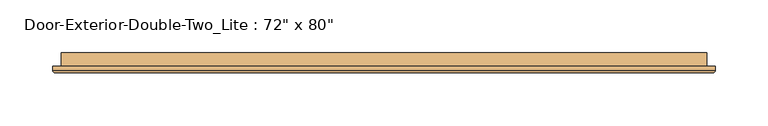
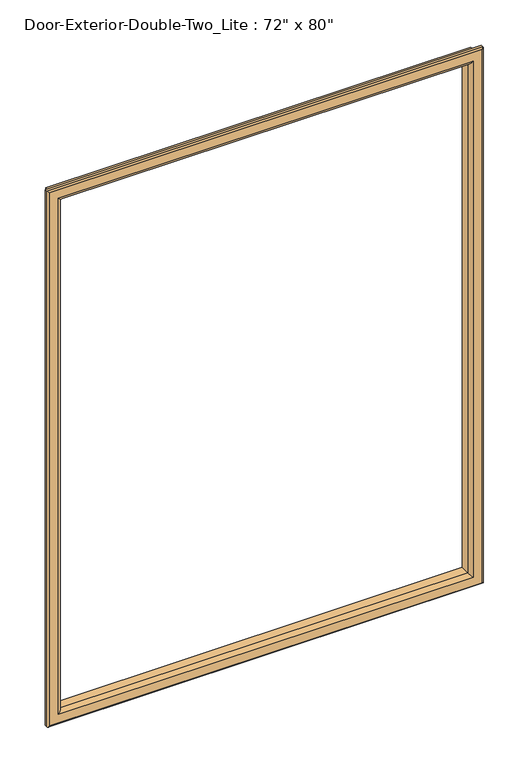
"""IFC4 building model written with IfcOpenShell, lengths in millimetres: door geometry."""

from ifc_helpers import new_model, si_unit, frame, origin, place, context, project, spatial, ellipse_curve, source, transform, mapped, element, save
from ifc_brep_helpers import plane_surface, cylinder_surface, advanced_brep


def door_3b4764fa(model_context):
    return source(origin(), model_context, "Body", "AdvancedBrep", [
        advanced_brep(
        [(-762.0, 47.625, 1117.6), (-762.0, 34.925, 1117.6), (-762.0, 34.925, 1914.525), (-762.0, 47.625, 1914.525), (-750.0, 33.925, 1129.6), (-750.0, 47.625, 1129.6), (-750.0, 47.625, 1902.525), (-750.0, 33.925, 1902.525), (-755.0, 28.925, 1124.6), (-755.0, 28.925, 1907.525), (-770.0, 30.925, 1109.6), (-768.0, 28.925, 1111.6), (-768.0, 28.925, 1920.525), (-770.0, 30.925, 1922.525), (-770.0, 34.925, 1109.6), (-770.0, 34.925, 1922.525), (-152.4, 34.925, 1914.525), (-152.4, 47.625, 1914.525), (-164.4, 47.625, 1902.525), (-164.4, 33.925, 1902.525), (-159.4, 28.925, 1907.525), (-146.4, 28.925, 1920.525), (-144.4, 30.925, 1922.525), (-144.4, 34.925, 1922.525), (-152.4, 34.925, 1117.6), (-152.4, 47.625, 1117.6), (-164.4, 47.625, 1129.6), (-164.4, 33.925, 1129.6), (-159.4, 28.925, 1124.6), (-146.4, 28.925, 1111.6), (-144.4, 30.925, 1109.6), (-144.4, 34.925, 1109.6)],
        [
            (0, 1),
            (1, 2),
            (2, 3),
            (3, 0),
            (4, 5),
            (5, 6),
            (6, 7),
            (7, 4),
            (8, 4, ellipse_curve(frame((-755.0, 33.925, 1124.6), z_axis=(-0.7071067811865475, 0.0, 0.7071067811865475), x_axis=(-0.7071067811865474, 0.0, -0.7071067811865476)), 7.0710678, 5.0)),
            (7, 9, ellipse_curve(frame((-755.0, 33.925, 1907.525), z_axis=(-0.7071067811865475, 0.0, -0.7071067811865475), x_axis=(0.7071067811865474, 0.0, -0.7071067811865476)), 7.0710678, 5.0)),
            (9, 8),
            (10, 11, ellipse_curve(frame((-768.0, 30.925, 1111.6), z_axis=(-0.7071067811865475, 0.0, 0.7071067811865475), x_axis=(-0.7071067811865474, 0.0, -0.7071067811865476)), 2.8284271, 2.0)),
            (11, 12),
            (12, 13, ellipse_curve(frame((-768.0, 30.925, 1920.525), z_axis=(-0.7071067811865475, 0.0, -0.7071067811865475), x_axis=(0.7071067811865474, 0.0, -0.7071067811865476)), 2.8284271, 2.0)),
            (13, 10),
            (14, 10),
            (13, 15),
            (15, 14),
            (2, 16),
            (16, 17),
            (17, 3),
            (6, 18),
            (18, 19),
            (19, 7),
            (19, 20, ellipse_curve(frame((-159.4, 33.925, 1907.525), z_axis=(-0.7071067811865475, 0.0, 0.7071067811865475), x_axis=(-0.7071067811865476, 0.0, -0.7071067811865474)), 7.0710678, 5.0)),
            (20, 9),
            (12, 21),
            (21, 22, ellipse_curve(frame((-146.4, 30.925, 1920.525), z_axis=(-0.7071067811865475, 0.0, 0.7071067811865475), x_axis=(-0.7071067811865476, 0.0, -0.7071067811865474)), 2.8284271, 2.0)),
            (22, 13),
            (22, 23),
            (23, 15),
            (16, 24),
            (24, 25),
            (25, 17),
            (18, 26),
            (26, 27),
            (27, 19),
            (27, 28, ellipse_curve(frame((-159.4, 33.925, 1124.6), z_axis=(0.7071067811865475, 0.0, 0.7071067811865475), x_axis=(-0.7071067811865474, 0.0, 0.7071067811865476)), 7.0710678, 5.0)),
            (28, 20),
            (21, 29),
            (29, 30, ellipse_curve(frame((-146.4, 30.925, 1111.6), z_axis=(0.7071067811865475, 0.0, 0.7071067811865475), x_axis=(-0.7071067811865474, 0.0, 0.7071067811865476)), 2.8284271, 2.0)),
            (30, 22),
            (30, 31),
            (31, 23),
            (31, 14),
            (1, 24),
            (0, 25),
            (5, 26),
            (4, 27),
            (8, 28),
            (11, 29),
            (10, 30),
        ],
        [
            plane_surface(frame((-762.0, 34.925, 1117.6), z_axis=(-1.0, 0.0, 0.0), x_axis=(0.0, 0.0, 1.0))),
            plane_surface(frame((-750.0, 47.625, 1129.6), z_axis=(1.0, 0.0, 0.0), x_axis=(0.0, 0.0, 1.0))),
            cylinder_surface(frame((-755.0, 33.925, 1117.6), z_axis=(0.0, 0.0, -1.0), x_axis=(-1.0, 0.0, 0.0)), 5.0),
            cylinder_surface(frame((-768.0, 30.925, 1117.6), z_axis=(0.0, 0.0, -1.0), x_axis=(-1.0, 0.0, 0.0)), 2.0),
            plane_surface(frame((-770.0, 30.925, 1109.6), z_axis=(-1.0, 0.0, 0.0), x_axis=(0.0, 0.0, 1.0))),
            plane_surface(frame((-762.0, 34.925, 1914.525), z_axis=(0.0, 0.0, 1.0), x_axis=(1.0, 0.0, 0.0))),
            plane_surface(frame((-750.0, 47.625, 1902.525), z_axis=(0.0, 0.0, -1.0), x_axis=(1.0, 0.0, 0.0))),
            cylinder_surface(frame((-762.0, 33.925, 1907.525), z_axis=(-1.0, 0.0, 0.0), x_axis=(0.0, 0.0, 1.0)), 5.0),
            cylinder_surface(frame((-762.0, 30.925, 1920.525), z_axis=(-1.0, 0.0, 0.0), x_axis=(0.0, 0.0, 1.0)), 2.0),
            plane_surface(frame((-770.0, 30.925, 1922.525), z_axis=(0.0, 0.0, 1.0), x_axis=(1.0, 0.0, 0.0))),
            plane_surface(frame((-152.4, 34.925, 1914.525), z_axis=(1.0, 0.0, 0.0), x_axis=(0.0, 0.0, -1.0))),
            plane_surface(frame((-164.4, 47.625, 1902.525), z_axis=(-1.0, 0.0, 0.0), x_axis=(0.0, 0.0, -1.0))),
            cylinder_surface(frame((-159.4, 33.925, 1914.525), z_axis=(0.0, 0.0, 1.0), x_axis=(1.0, 0.0, 0.0)), 5.0),
            cylinder_surface(frame((-146.4, 30.925, 1914.525), z_axis=(0.0, 0.0, 1.0), x_axis=(1.0, 0.0, 0.0)), 2.0),
            plane_surface(frame((-144.4, 30.925, 1922.525), z_axis=(1.0, 0.0, 0.0), x_axis=(0.0, 0.0, -1.0))),
            plane_surface(frame((-144.4, 34.925, 1109.6), z_axis=(0.0, 1.0, 0.0), x_axis=(-1.0, 0.0, 0.0))),
            plane_surface(frame((-152.4, 34.925, 1117.6), z_axis=(0.0, 0.0, -1.0), x_axis=(-1.0, 0.0, 0.0))),
            plane_surface(frame((-152.4, 47.625, 1117.6), z_axis=(0.0, 1.0, 0.0), x_axis=(-1.0, 0.0, 0.0))),
            plane_surface(frame((-164.4, 47.625, 1129.6), z_axis=(0.0, 0.0, 1.0), x_axis=(-1.0, 0.0, 0.0))),
            cylinder_surface(frame((-152.4, 33.925, 1124.6), z_axis=(1.0, 0.0, 0.0), x_axis=(0.0, 0.0, -1.0)), 5.0),
            plane_surface(frame((-159.4, 28.925, 1124.6), z_axis=(0.0, -1.0, 0.0), x_axis=(-1.0, 0.0, 0.0))),
            cylinder_surface(frame((-152.4, 30.925, 1111.6), z_axis=(1.0, 0.0, 0.0), x_axis=(0.0, 0.0, -1.0)), 2.0),
            plane_surface(frame((-144.4, 30.925, 1109.6), z_axis=(0.0, 0.0, -1.0), x_axis=(-1.0, 0.0, 0.0))),
        ],
        [
            (0, [[1, 2, 3, 4]]),
            (1, [[5, 6, 7, 8]]),
            (2, [[9, -8, 10, 11]]),
            (3, [[12, 13, 14, 15]]),
            (4, [[16, -15, 17, 18]]),
            (5, [[-3, 19, 20, 21]]),
            (6, [[-7, 22, 23, 24]]),
            (7, [[-10, -24, 25, 26]]),
            (8, [[-14, 27, 28, 29]]),
            (9, [[-17, -29, 30, 31]]),
            (10, [[-20, 32, 33, 34]]),
            (11, [[-23, 35, 36, 37]]),
            (12, [[-25, -37, 38, 39]]),
            (13, [[-28, 40, 41, 42]]),
            (14, [[-30, -42, 43, 44]]),
            (15, [[-31, -44, 45, -18], [46, -32, -19, -2]]),
            (16, [[-33, -46, -1, 47]]),
            (17, [[-21, -34, -47, -4], [48, -35, -22, -6]]),
            (18, [[-36, -48, -5, 49]]),
            (19, [[-38, -49, -9, 50]]),
            (20, [[51, -40, -27, -13], [-26, -39, -50, -11]]),
            (21, [[-41, -51, -12, 52]]),
            (22, [[-43, -52, -16, -45]]),
        ],
    ),
    ])


if __name__ == "__main__":
    model = new_model("IFC4")
    model_context = context("Model", 3, world=origin())
    ifc_project = project(units=[si_unit("LENGTHUNIT", "METRE", prefix="MILLI")], contexts=[model_context])
    site = spatial("IfcSite", under=ifc_project)
    building = spatial("IfcBuilding", under=site)
    placement = place(None, origin())
    door_shape = door_3b4764fa(model_context)
    element("IfcDoor", 1, ObjectType="Door-Exterior-Double-Two_Lite : 72\" x 80\"", at=placement, inside=building, context=model_context, shape_type="MappedRepresentation", body=[
        mapped(door_shape, transform((0.0, 0.0, 0.0), x_axis=(1.0, 0.0, 0.0), y_axis=(0.0, 1.0, 0.0), z_axis=(0.0, 0.0, 1.0))),
    ])
    save(model, "model.ifc")

# Revit data of these elements
# Type "Door-Exterior-Double-Two_Lite : 72\" x 80\""
#   Type Mark = "18"
#   Assembly Code = "B2030100"
#   Analytic Construction = "Metal frame, double glass door"
#   Top Rail = 0' - 4 5/8"
#   Threshold Length [instance default] = 6' - 4"
#   Threshold Offset [instance default] = 0' - 0 1/2"
#   Thickness = 0' - 1 3/4"
#   Thermal Resistance (R) = 0.242926 (m²·K)/W
#   Swing Angle [instance default] = 90.00°
#   Strike Height = 3' - 4"
#   Stiles = 0' - 6"
#   SinglePanelWidth = 3' - 0"
#   Rough Width [instance default] = 6' - 4"
#   Rough Height [instance default] = 7' - 0"
#   MFOpeningHeight [instance default] = 0' - 4"
#   MFOpeningWidth [instance default] = 0' - 4"
#   Lock Rail = 0' - 8"
#   Inset Calculate [instance default] = 0' - 4"
#   Masonry Inset [instance default] = 0' - 1"
#   Height = 6' - 8"
#   Width = 6' - 0"
#   Heat Transfer Coefficient (U) = 4.11674 W/(m²·K)
#   Glass Thickness = 0' - 0 3/4"
#   Masonry Frame Depth = 0' - 5 3/4"
#   Bottom Rail = 0' - 10"
#   Threshold [instance default] = yes
#   Masonry Frame [instance default] = yes
#   Function = 1
#   Dry Wall Frame [instance default] = no
#   Threshold Material = none
#   Panic Bar Material = Metal - Stainless Steel
#   Panel Material = Metal - Painted - Grey
#   Glass Stop Material = Metal - Painted - Grey
#   Frame Material = Metal - Painted - Grey
#   Exterior Pull Material = Metal - Stainless Steel
#   Visual Light Transmittance = 0
#   Solar Heat Gain Coefficient = 0
#   Wall Closure = (empty or 0)
# Element 1 (IfcDoor, "Door-Exterior-Double-Two_Lite : 72\" x 80\"")
#   Inset Calculate = 0' - 2 1/2"
#   Masonry Inset = -0' - 0 1/2"
#   Materials on its faces: "Metal - Painted - Grey", "Metal - Stainless Steel", "Glass"
# Materials
#   "Metal - Stainless Steel": class "Metal", colour RGB 247 247 247, transparency 0
#   "Metal - Painted - Grey": class "Paint", colour RGB 104 104 104, transparency 0, Cost = 0
#   "Glass": class "Glass", colour RGB 218 227 224, transparency 0.85, Description = "Soda Lime Glass", Cost = 0
